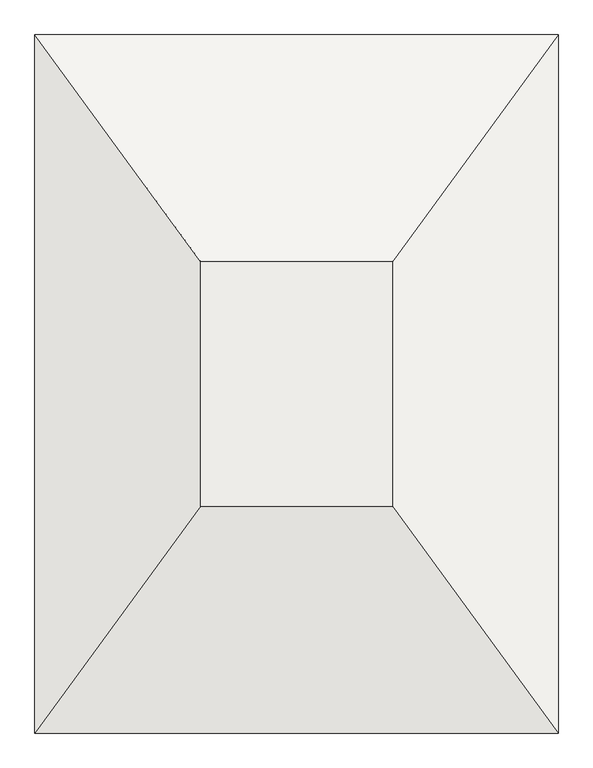
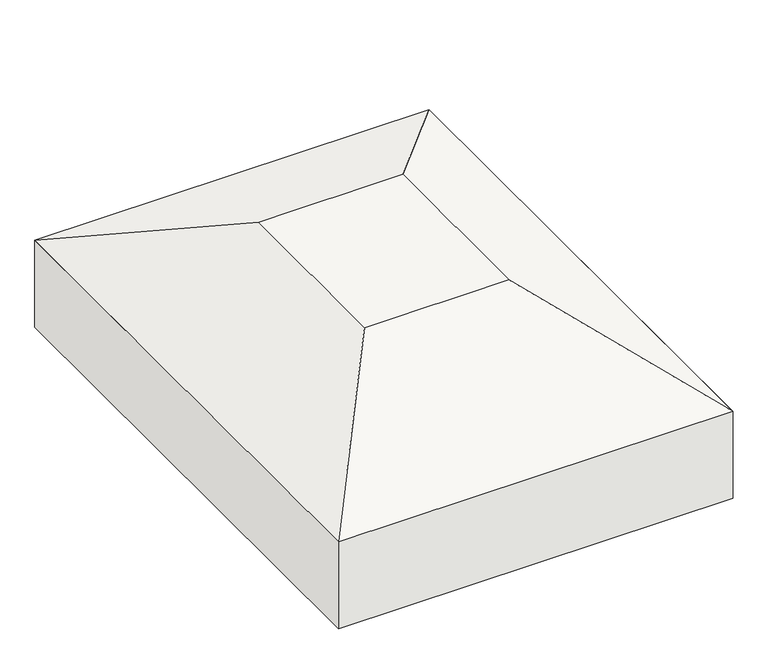
"""IFC4 building model written with IfcOpenShell, lengths in millimetres: slab geometry, 独立基础 - 坡形截面 : 独立基础 - 坡形截面."""

from ifc_helpers import new_model, si_unit, frame, origin, place, context, project, spatial, polyline, outline, extrude, faceted_brep, source, transform, mapped, element, save


def slab_86cecf96(model_context):
    return source(origin(), model_context, "Body", "SolidModel", [
        faceted_brep([(750.0, 1000.0, -300.0), (750.0, -1000.0, -300.0), (-750.0, -1000.0, -300.0), (-750.0, 1000.0, -300.0), (275.0, 350.0, 0.0), (-275.0, 350.0, 0.0), (-275.0, -350.0, 0.0), (275.0, -350.0, 0.0)], [[[0, 1, 2, 3]], [[4, 5, 6, 7]], [[5, 4, 0, 3]], [[6, 5, 3, 2]], [[7, 6, 2, 1]], [[4, 7, 1, 0]]]),
        extrude(outline(polyline([(750.0, 1000.0), (750.0, -1000.0), (-750.0, -1000.0), (-750.0, 1000.0), (750.0, 1000.0)])), frame((0.0, 0.0, -650.0), z_axis=(0.0, 0.0, 1.0), x_axis=(1.0, 0.0, 0.0)), (0.0, 0.0, 1.0), 350.0),
    ])


if __name__ == "__main__":
    model = new_model("IFC4")
    model_context = context("Model", 3, world=origin())
    ifc_project = project(units=[si_unit("LENGTHUNIT", "METRE", prefix="MILLI")], contexts=[model_context])
    site = spatial("IfcSite", under=ifc_project)
    building = spatial("IfcBuilding", under=site)
    placement = place(None, origin())
    slab_shape = slab_86cecf96(model_context)
    element("IfcSlab", 1, ObjectType="独立基础 - 坡形截面 : 独立基础 - 坡形截面", at=placement, inside=building, context=model_context, shape_type="MappedRepresentation", body=[
        mapped(slab_shape, transform((0.0, 0.0, 0.0), x_axis=(1.0, 0.0, 0.0), y_axis=(0.0, 1.0, 0.0), z_axis=(0.0, 0.0, 1.0))),
    ])
    save(model, "model.ifc")

# Revit data of these elements
# Type "独立基础 - 坡形截面 : 独立基础 - 坡形截面"
#   h2 = 300 mm
#   h1 = 350 mm
#   d2 = 50 mm
#   d1 = 50 mm
#   Width = 1500 mm
#   Length = 2000 mm
#   Hc = 600 mm
#   Foundation Thickness = 650 mm
#   Bc = 450 mm
#   Structural Material [instance default] = 混凝土 - 现场浇注混凝土
#   Assembly Code = ""
# Element 1 (IfcSlab, "独立基础 - 坡形截面 : 独立基础 - 坡形截面")
#   Materials on its faces: "混凝土 - 现场浇注混凝土"
# Materials
#   "混凝土 - 现场浇注混凝土": class "混凝土", colour RGB 192 192 192, transparency 0
